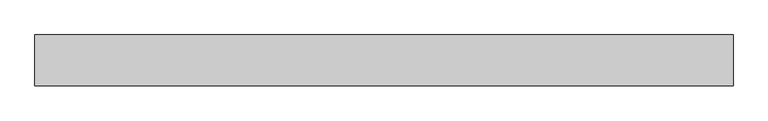
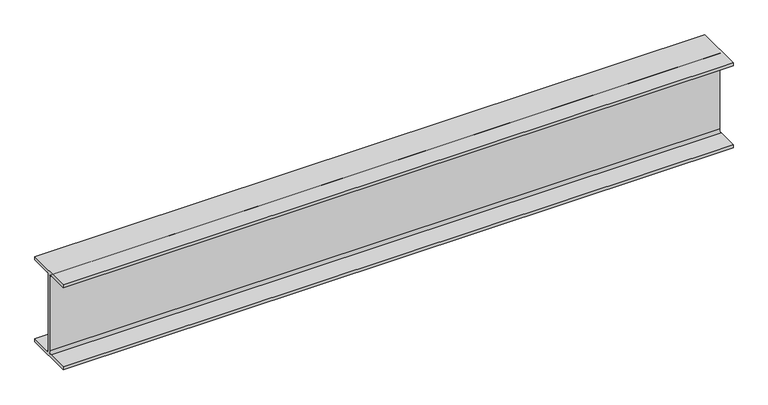
"""IFC4 building model written with IfcOpenShell, lengths in millimetres: beam geometry, Old_Steel Beam_H-KSD3502 : H_SB_ASB_H-200×200x8x12."""

import ifcopenshell
import ifcopenshell.guid

model = None  # the IFC model being written
_history = None  # IfcOwnerHistory: only IFC2X3 demands one
_inside = {}  # id of a spatial element -> (the spatial element, [elements in it])
_under = {}  # id of a project, library or spatial element -> (it, [spatial elements below it])
_declared = {}  # id of a project -> (the project, [libraries it declares])
_typed = {}  # id of a type object -> (the type object, [elements of that type])
_made_of = {}  # id of a material, layer set ... -> (it, [elements and type objects made of it])


def new_model(schema):
    """Start an empty IFC model of exactly this schema.

    Asked for "IFC4X3", IfcOpenShell would pick the latest addendum, in which some entities
    have other attributes; the version numbers below select the first issue.
    IFC2X3 requires an IfcOwnerHistory on every rooted entity: one is made here for all.
    """
    global model, _history
    if schema == "IFC4X3":
        model = ifcopenshell.file(schema_version=(4, 3, 0, 0))
    else:
        model = ifcopenshell.file(schema=schema)
    _inside.clear()
    _under.clear()
    _declared.clear()
    _typed.clear()
    _made_of.clear()
    _history = None
    if model.schema == "IFC2X3":
        org = make("IfcOrganization", Name="unknown")
        user = make(
            "IfcPersonAndOrganization",
            ThePerson=make("IfcPerson", FamilyName="unknown"),
            TheOrganization=org,
        )
        app = make(
            "IfcApplication",
            ApplicationDeveloper=org,
            Version="unknown",
            ApplicationFullName="unknown",
            ApplicationIdentifier="unknown",
        )
        _history = make(
            "IfcOwnerHistory",
            OwningUser=user,
            OwningApplication=app,
            ChangeAction="ADDED",
            CreationDate=0,
        )
    return model


def make(cls, **values):
    """One entity of the class cls with the attributes given. An attribute that is None is left unset."""
    return model.create_entity(
        cls, **{name: value for name, value in values.items() if value is not None}
    )


def rooted(cls, **values):
    """An entity with a GlobalId (a new one), such as an element, a storey or a relation."""
    return make(cls, GlobalId=ifcopenshell.guid.new(), OwnerHistory=_history, **values)


def si_unit(unit_type, name, prefix=None):
    """IfcSIUnit, for example si_unit("LENGTHUNIT", "METRE", prefix="MILLI")."""
    return make("IfcSIUnit", UnitType=unit_type, Prefix=prefix, Name=name)


def assignment(units):
    """IfcUnitAssignment: the units of a project."""
    return None if units is None else make("IfcUnitAssignment", Units=units)


def point(xyz):
    """IfcCartesianPoint."""
    return None if xyz is None else make("IfcCartesianPoint", Coordinates=xyz)


def direction(xyz):
    """IfcDirection."""
    return None if xyz is None else make("IfcDirection", DirectionRatios=xyz)


def frame(location, z_axis=None, x_axis=None):
    """IfcAxis2Placement3D, a coordinate frame: its origin and axes. An axis left out is left unset."""
    return make(
        "IfcAxis2Placement3D",
        Location=point(location),
        Axis=direction(z_axis),
        RefDirection=direction(x_axis),
    )


def frame_2d(location, x_axis=None):
    """IfcAxis2Placement2D, a coordinate frame in the plane: its origin and x axis."""
    return make(
        "IfcAxis2Placement2D", Location=point(location), RefDirection=direction(x_axis)
    )


def origin():
    """The frame at (0, 0, 0) with its axes left unset."""
    return frame((0.0, 0.0, 0.0))


def place(relative_to, where):
    """IfcLocalPlacement: puts the frame where relative to a parent placement (None: the world)."""
    return make(
        "IfcLocalPlacement", PlacementRelTo=relative_to, RelativePlacement=where
    )


def context(
    kind, dimensions, precision=None, world=None, true_north=None, identifier=None
):
    """IfcGeometricRepresentationContext, for example the 3D "Model" context."""
    return make(
        "IfcGeometricRepresentationContext",
        ContextIdentifier=identifier,
        ContextType=kind,
        CoordinateSpaceDimension=dimensions,
        Precision=precision,
        WorldCoordinateSystem=world,
        TrueNorth=true_north,
    )


def project(units=None, contexts=None):
    """IfcProject with its units and contexts."""
    return rooted(
        "IfcProject",
        Name="project",
        RepresentationContexts=contexts,
        UnitsInContext=assignment(units),
    )


def spatial(cls, under=None, at=None, **own):
    """A site, building, storey or space (cls), placed at a placement, below another one or the project."""
    s = rooted(cls, ObjectPlacement=at, **own)
    if under is not None:
        _under.setdefault(under.id(), (under, []))[1].append(s)
    return s


def polyline(points):
    """IfcPolyline through the points."""
    return make("IfcPolyline", Points=[point(p) for p in points])


def circle_curve(where, radius):
    """IfcCircle in the frame where."""
    return make("IfcCircle", Position=where, Radius=radius)


def trimmed(basis, trim1, trim2, sense, master):
    """IfcTrimmedCurve: the piece of a basis curve between two trims."""
    return make(
        "IfcTrimmedCurve",
        BasisCurve=basis,
        Trim1=trim1,
        Trim2=trim2,
        SenseAgreement=sense,
        MasterRepresentation=master,
    )


def segment(curve, same_sense, transition):
    """IfcCompositeCurveSegment."""
    return make(
        "IfcCompositeCurveSegment",
        Transition=transition,
        SameSense=same_sense,
        ParentCurve=curve,
    )


def composite_curve(segments, self_intersect=None):
    """IfcCompositeCurve: segments joined end to end."""
    return make("IfcCompositeCurve", Segments=segments, SelfIntersect=self_intersect)


def outline(outer, holes=None, kind="AREA"):
    """IfcArbitraryClosedProfileDef: a profile drawn as a closed curve; with holes, ...WithVoids."""
    if holes is None:
        return make("IfcArbitraryClosedProfileDef", ProfileType=kind, OuterCurve=outer)
    return make(
        "IfcArbitraryProfileDefWithVoids",
        ProfileType=kind,
        OuterCurve=outer,
        InnerCurves=holes,
    )


def extrude(swept, where, along, depth):
    """IfcExtrudedAreaSolid: the profile swept, set in the frame where, extruded along a direction by depth."""
    return make(
        "IfcExtrudedAreaSolid",
        SweptArea=swept,
        Position=where,
        ExtrudedDirection=direction(along),
        Depth=depth,
    )


def shape(context_of_items, identifier, shape_type, items):
    """IfcShapeRepresentation: the items that make up one representation, for example the "Body"."""
    return make(
        "IfcShapeRepresentation",
        ContextOfItems=context_of_items,
        RepresentationIdentifier=identifier,
        RepresentationType=shape_type,
        Items=items,
    )


def source(mapping_origin, context_of_items, identifier, shape_type, items):
    """IfcRepresentationMap: a shape defined once, which mapped items show again and again."""
    return make(
        "IfcRepresentationMap",
        MappingOrigin=mapping_origin,
        MappedRepresentation=shape(context_of_items, identifier, shape_type, items),
    )


def transform(
    local_origin,
    x_axis=None,
    y_axis=None,
    z_axis=None,
    scale=None,
    scale2=None,
    scale3=None,
    uniform=True,
):
    """IfcCartesianTransformationOperator3D, or its non-uniform kind. x_axis, y_axis, z_axis: its Axis1, 2, 3."""
    if uniform:
        return make(
            "IfcCartesianTransformationOperator3D",
            Axis1=direction(x_axis),
            Axis2=direction(y_axis),
            LocalOrigin=point(local_origin),
            Scale=scale,
            Axis3=direction(z_axis),
        )
    return make(
        "IfcCartesianTransformationOperator3DnonUniform",
        Axis1=direction(x_axis),
        Axis2=direction(y_axis),
        LocalOrigin=point(local_origin),
        Scale=scale,
        Axis3=direction(z_axis),
        Scale2=scale2,
        Scale3=scale3,
    )


def mapped(mapping_source, mapping_target):
    """IfcMappedItem: shows the shape of a source again, moved by a transform."""
    return make(
        "IfcMappedItem", MappingSource=mapping_source, MappingTarget=mapping_target
    )


def made_of(thing, what):
    """Note that an element or type object is made of a material, layer set ...; save() writes the relation."""
    if what is not None:
        _made_of.setdefault(what.id(), (what, []))[1].append(thing)
    return thing


def element(
    cls,
    number,
    at=None,
    inside=None,
    cuts=None,
    type_object=None,
    material=None,
    context=None,
    identifier="Body",
    shape_type=None,
    held_by="IfcProductDefinitionShape",
    body=None,
    shapes=None,
    **own,
):
    """One element of the class cls, such as IfcWall. Its Tag is "e" and its number.

    at: its placement. inside: the storey or other place that contains it. cuts: it is an
    opening in that element (IfcRelVoidsElement). A single representation is given by context,
    identifier, shape_type and body (its items); several are given by shapes. held_by: the class
    of the entity that holds the representations. save() writes the other relations.
    """
    e = rooted(cls, Tag="e%d" % number, ObjectPlacement=at, **own)
    if body is not None:
        shapes = [shape(context, identifier, shape_type, body)]
    if shapes is not None:
        e.Representation = make(held_by, Representations=shapes)
    if inside is not None:
        _inside.setdefault(inside.id(), (inside, []))[1].append(e)
    if cuts is not None:
        rooted(
            "IfcRelVoidsElement", RelatingBuildingElement=cuts, RelatedOpeningElement=e
        )
    if type_object is not None:
        _typed.setdefault(type_object.id(), (type_object, []))[1].append(e)
    return made_of(e, material)


def aggregate(whole, parts):
    """IfcRelAggregates: a whole, such as a stair, and the parts it consists of."""
    return rooted("IfcRelAggregates", RelatingObject=whole, RelatedObjects=parts)


def save(model, path):
    """Write the relations noted so far, then the file.

    IfcRelAggregates (storeys below a building ...), IfcRelContainedInSpatialStructure (elements
    in a storey), IfcRelDefinesByType, IfcRelAssociatesMaterial and IfcRelDeclares: one each for
    every whole, place, type object, material and project.
    """
    for whole, parts in _under.values():
        aggregate(whole, parts)
    for where, things in _inside.values():
        rooted(
            "IfcRelContainedInSpatialStructure",
            RelatedElements=things,
            RelatingStructure=where,
        )
    for kind, things in _typed.values():
        rooted("IfcRelDefinesByType", RelatedObjects=things, RelatingType=kind)
    for what, things in _made_of.values():
        rooted("IfcRelAssociatesMaterial", RelatedObjects=things, RelatingMaterial=what)
    for by, libraries in _declared.values():
        rooted("IfcRelDeclares", RelatingContext=by, RelatedDefinitions=libraries)
    model.write(path)


def beam_9b741c7f(model_context):
    return source(origin(), model_context, "Body", "SweptSolid", [
        extrude(outline(composite_curve([segment(polyline([(82.5, -141.5), (82.5, -151.7), (-82.5, -151.7), (-82.5, -141.5), (-11.9, -141.5)]), True, "CONTINUOUS"), segment(trimmed(circle_curve(frame_2d((-11.9, -132.6)), 8.9), [point((-11.9, -141.5))], [point((-3.0, -132.6))], True, "CARTESIAN"), True, "CONTINUOUS"), segment(polyline([(-3.0, -132.6), (-3.0, 132.6)]), True, "CONTINUOUS"), segment(trimmed(circle_curve(frame_2d((-11.9, 132.6)), 8.9), [point((-3.0, 132.6))], [point((-11.9, 141.5))], True, "CARTESIAN"), True, "CONTINUOUS"), segment(polyline([(-11.9, 141.5), (-82.5, 141.5), (-82.5, 151.7), (82.5, 151.7), (82.5, 141.5), (11.9, 141.5)]), True, "CONTINUOUS"), segment(trimmed(circle_curve(frame_2d((11.9, 132.6)), 8.9), [point((11.9, 141.5))], [point((3.0, 132.6))], True, "CARTESIAN"), True, "CONTINUOUS"), segment(polyline([(3.0, 132.6), (3.0, -132.6)]), True, "CONTINUOUS"), segment(trimmed(circle_curve(frame_2d((11.9, -132.6)), 8.9), [point((3.0, -132.6))], [point((11.9, -141.5))], True, "CARTESIAN"), True, "CONTINUOUS"), segment(polyline([(11.9, -141.5), (82.5, -141.5)]), True, "CONTINUOUS")], self_intersect=False)), frame((-1289.752068, 0.0, 0.0), z_axis=(1.0, 0.0, 0.0), x_axis=(0.0, 1.0, 0.0)), (0.0, 0.0, 1.0), 2265.6401913),
    ])


if __name__ == "__main__":
    model = new_model("IFC4")
    model_context = context("Model", 3, world=origin())
    ifc_project = project(units=[si_unit("LENGTHUNIT", "METRE", prefix="MILLI")], contexts=[model_context])
    site = spatial("IfcSite", under=ifc_project)
    building = spatial("IfcBuilding", under=site)
    placement = place(None, origin())
    beam_shape = beam_9b741c7f(model_context)
    element("IfcBeam", 1, ObjectType="Old_Steel Beam_H-KSD3502 : H_SB_ASB_H-200×200x8x12", at=placement, inside=building, context=model_context, shape_type="MappedRepresentation", body=[
        mapped(beam_shape, transform((0.0, 0.0, 0.0), x_axis=(1.0, 0.0, 0.0), y_axis=(0.0, 1.0, 0.0), z_axis=(0.0, 0.0, 1.0))),
    ])
    save(model, "model.ifc")

# Revit data of these elements
# Type "Old_Steel Beam_H-KSD3502 : H_SB_ASB_H-200×200x8x12"
#   Width = 20.0 cm
#   Web Thickness = 0.8 cm
#   Web Fillet = 1.3 cm
#   Warping Constant = 141376.0 cm⁶
#   Torsional Moment of Inertia = 26.2485 cm⁴
#   Torsional Modulus = 1.0 cm³
#   Section Area = 63.53 cm²
#   Plastic Modulus weak axis = 244.0 cm³
#   Plastic Modulus strong axis = 525.0 cm³
#   Perimeter = 1.16 m²/m
#   Nominal Weight = 49.90 kgf/m
#   Moment of Inertia weak axis = 1600.00 cm⁴
#   Moment of Inertia strong axis = 4720.00 cm⁴
#   Height = 20.0 cm
#   Flange Thickness = 1.2 cm
#   Elastic Modulus weak axis = 160.0 cm³
#   Elastic Modulus strong axis = 472.0 cm³
#   Centroid Vertical = 10.0 cm
#   Centroid Horizontal = 10.0 cm
#   Length [instance default] = 1.5240 m
#   Structural Material [instance default] = Steel, 45-345
#   Assembly Code = ""
# Element 1 (IfcBeam, "Old_Steel Beam_H-KSD3502 : H_SB_ASB_H-200×200x8x12")
#   Structural Material = none
# Materials
#   "Steel, 45-345": class "Metal", colour RGB 189 187 185, transparency 0, Description = "Steel 345 MPa", Cost = 0
